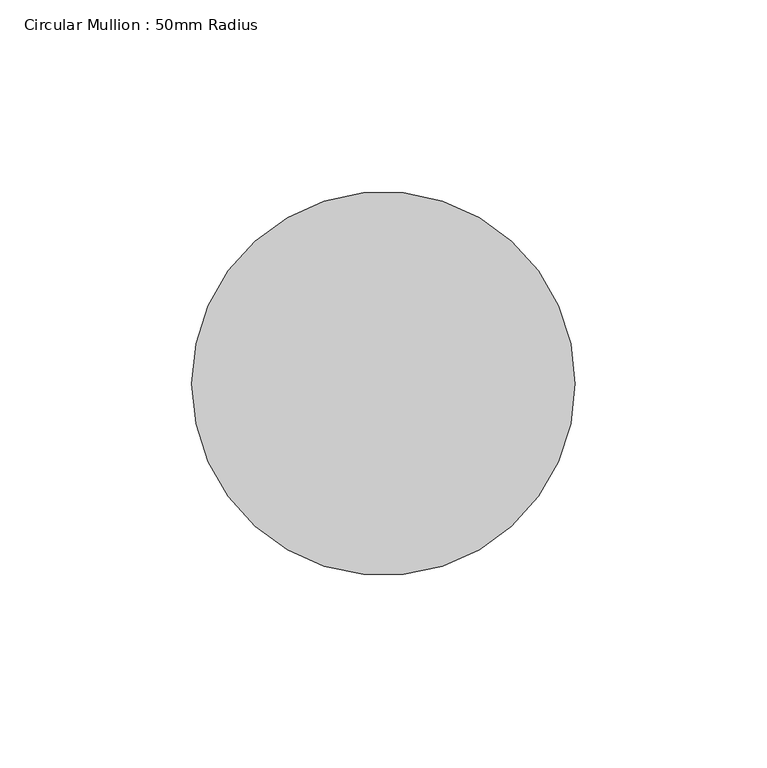
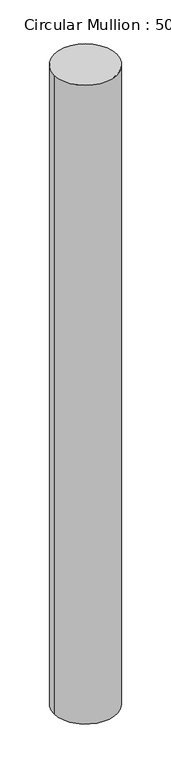
"""IFC4 building model written with IfcOpenShell, lengths in millimetres: member geometry, Circular Mullion : 50mm Radius."""

from ifc_helpers import new_model, si_unit, point, frame, origin, origin_2d, place, context, project, spatial, circle_curve, trimmed, segment, composite_curve, outline, extrude, source, transform, mapped, element, save


def circular_mullion_50mm_radius_d72c355f(model_context):
    return source(origin(), model_context, "Body", "SweptSolid", [
        extrude(outline(composite_curve([segment(trimmed(circle_curve(origin_2d(), 50.0), [point((50.0, 0.0))], [point((-50.0, 0.0))], False, "CARTESIAN"), True, "CONTINUOUS"), segment(trimmed(circle_curve(origin_2d(), 50.0), [point((-50.0, 0.0))], [point((50.0, 0.0))], False, "CARTESIAN"), True, "CONTINUOUS")], self_intersect=False)), frame((0.0, 0.0, -1076.1673713), z_axis=(0.0, 0.0, 1.0), x_axis=(1.0, 0.0, 0.0)), (0.0, 0.0, 1.0), 1076.1673713),
    ])


if __name__ == "__main__":
    model = new_model("IFC4")
    model_context = context("Model", 3, world=origin())
    ifc_project = project(units=[si_unit("LENGTHUNIT", "METRE", prefix="MILLI")], contexts=[model_context])
    site = spatial("IfcSite", under=ifc_project)
    building = spatial("IfcBuilding", under=site)
    placement = place(None, origin())
    circular_mullion_50mm_radius_shape = circular_mullion_50mm_radius_d72c355f(model_context)
    element("IfcMember", 1, ObjectType="Circular Mullion : 50mm Radius", at=placement, inside=building, context=model_context, shape_type="MappedRepresentation", body=[
        mapped(circular_mullion_50mm_radius_shape, transform((0.0, 0.0, 0.0), x_axis=(1.0, 0.0, 0.0), y_axis=(0.0, 1.0, 0.0), z_axis=(0.0, 0.0, 1.0))),
    ])
    save(model, "model.ifc")

# Revit data of these elements
# Type "Circular Mullion : 50mm Radius"
#   built-in parameter 1007350 = 0.164042 (stored number, unit not read)
# Element 1 (IfcMember, "Circular Mullion : 50mm Radius")
#   Materials on its faces: "Aluminium"
# Materials
#   "Aluminium": class "Metal", colour RGB 247 247 247, transparency 0, Description = "Aluminium 6061", Cost = 0
